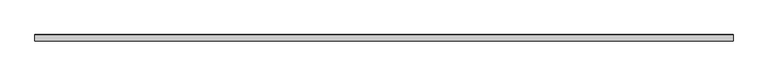
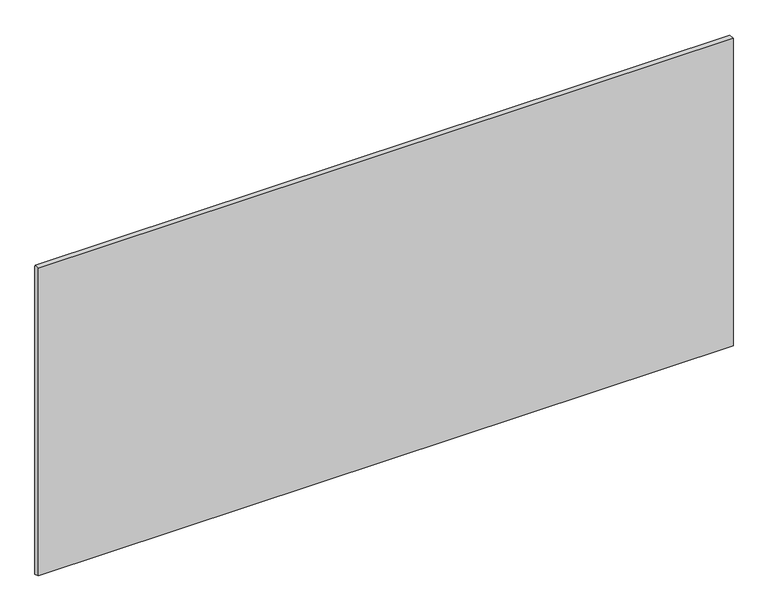
"""IFC4 building model written with IfcOpenShell, lengths in millimetres: proxy geometry, Stucco008 1210 : Stucco008 1210."""

from ifc_helpers import new_model, si_unit, frame, origin, place, context, project, spatial, polyline, outline, extrude, source, transform, mapped, element, save


def generic_models_c428cdc5(model_context):
    return source(origin(), model_context, "Body", "SweptSolid", [
        extrude(outline(polyline([(9757.0074636, 36545.734375), (9757.0074636, 37481.0682812), (9773.5175834, 37481.0682812), (9773.5175834, 37477.5884812), (9774.7875834, 37477.5884812), (9774.7875834, 36540.0208437), (9757.0074636, 36545.734375)])), frame((3694.2883192, 0.0, 0.0), z_axis=(1.0, 0.0, 0.0), x_axis=(0.0, 1.0, 0.0)), (0.0, 0.0, 1.0), 2000.0),
    ])


if __name__ == "__main__":
    model = new_model("IFC4")
    model_context = context("Model", 3, world=origin())
    ifc_project = project(units=[si_unit("LENGTHUNIT", "METRE", prefix="MILLI")], contexts=[model_context])
    site = spatial("IfcSite", under=ifc_project)
    building = spatial("IfcBuilding", under=site)
    placement = place(None, origin())
    generic_models_shape = generic_models_c428cdc5(model_context)
    element("IfcBuildingElementProxy", 1, Name="Stucco008 1210 : Stucco008 1210", ObjectType="Stucco008 1210 : Stucco008 1210", at=placement, inside=building, context=model_context, shape_type="MappedRepresentation", body=[
        mapped(generic_models_shape, transform((0.0, 0.0, 0.0), x_axis=(1.0, 0.0, 0.0), y_axis=(0.0, 1.0, 0.0), z_axis=(0.0, 0.0, 1.0))),
    ])
    save(model, "model.ifc")

# Revit data of these elements
# Type "Stucco008 1210 : Stucco008 1210"
#   NameOverride = "Stucco008"
# Element 1 (IfcBuildingElementProxy, "Stucco008 1210 : Stucco008 1210")
#   Materials on its faces: "7/8\" SMOOTH TROWEL EXTERIOR STUCCO"
# Materials
#   "7/8\" SMOOTH TROWEL EXTERIOR STUCCO": class "Unassigned", colour RGB 255 255 255, transparency 0, Cost = 0
